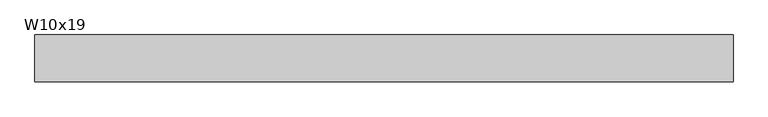
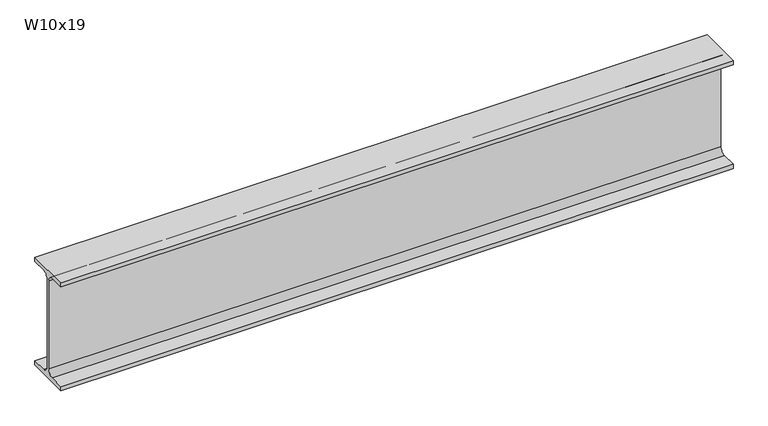
"""IFC4 building model written with IfcOpenShell, lengths in millimetres: beam geometry, RME W-Wide Flange : W10x19."""

from ifc_helpers import new_model, si_unit, point, frame, frame_2d, origin, place, context, project, spatial, polyline, circle_curve, trimmed, segment, composite_curve, outline, extrude, source, transform, mapped, element, save


def w10x19_decb9594(model_context):
    return source(origin(), model_context, "Body", "SweptSolid", [
        extrude(outline(composite_curve([segment(polyline([(51.054, -119.507), (51.054, -129.54), (-51.054, -129.54), (-51.054, -119.507), (-16.9545, -119.507)]), True, "CONTINUOUS"), segment(trimmed(circle_curve(frame_2d((-16.9545, -105.7275)), 13.7795), [point((-16.9545, -119.507))], [point((-3.175, -105.7275))], True, "CARTESIAN"), True, "CONTINUOUS"), segment(polyline([(-3.175, -105.7275), (-3.175, 105.7275)]), True, "CONTINUOUS"), segment(trimmed(circle_curve(frame_2d((-16.9545, 105.7275)), 13.7795), [point((-3.175, 105.7275))], [point((-16.9545, 119.507))], True, "CARTESIAN"), True, "CONTINUOUS"), segment(polyline([(-16.9545, 119.507), (-51.054, 119.507), (-51.054, 129.54), (51.054, 129.54), (51.054, 119.507), (16.9545, 119.507)]), True, "CONTINUOUS"), segment(trimmed(circle_curve(frame_2d((16.9545, 105.7275)), 13.7795), [point((16.9545, 119.507))], [point((3.175, 105.7275))], True, "CARTESIAN"), True, "CONTINUOUS"), segment(polyline([(3.175, 105.7275), (3.175, -105.7275)]), True, "CONTINUOUS"), segment(trimmed(circle_curve(frame_2d((16.9545, -105.7275)), 13.7795), [point((3.175, -105.7275))], [point((16.9545, -119.507))], True, "CARTESIAN"), True, "CONTINUOUS"), segment(polyline([(16.9545, -119.507), (51.054, -119.507)]), True, "CONTINUOUS")], self_intersect=False)), frame((-763.2780813, 0.0, 0.0), z_axis=(1.0, 0.0, 0.0), x_axis=(0.0, 1.0, 0.0)), (0.0, 0.0, 1.0), 1526.5561627),
    ])


if __name__ == "__main__":
    model = new_model("IFC4")
    model_context = context("Model", 3, world=origin())
    ifc_project = project(units=[si_unit("LENGTHUNIT", "METRE", prefix="MILLI")], contexts=[model_context])
    site = spatial("IfcSite", under=ifc_project)
    building = spatial("IfcBuilding", under=site)
    placement = place(None, origin())
    w10x19_shape = w10x19_decb9594(model_context)
    element("IfcBeam", 1, ObjectType="RME W-Wide Flange : W10x19", at=placement, inside=building, context=model_context, shape_type="MappedRepresentation", body=[
        mapped(w10x19_shape, transform((0.0, 0.0, 0.0), x_axis=(1.0, 0.0, 0.0), y_axis=(0.0, 1.0, 0.0), z_axis=(0.0, 0.0, 1.0))),
    ])
    save(model, "model.ifc")

# Revit data of these elements
# Type "RME W-Wide Flange : W10x19"
#   WELD P [instance default] = ""
#   WELD LE [instance default] = ""
#   WELD D [instance default] = ""
#   TOP SECTION SIZE [instance default] = ""
#   TOP SECTION LENGTH [instance default] = ""
#   REMARKS [instance default] = ""
#   REINF TYPE [instance default] = ""
#   Nominal Size = "W24"
#   End Bearing Capacity [instance default] = ""
#   BOT SECTION SIZE [instance default] = ""
#   BOT SECTION LENGTH [instance default] = ""
#   Assembly Code = "B10"
#   W = 19
#   Start Extension Calculation [instance default] = 10' - 0"
#   Start Extension [instance default] = -0' - 0 1/2"
#   End Extension Calculation [instance default] = 10' - 0"
#   End Extension [instance default] = -0' - 0 1/2"
#   Length [instance default] = 5' - 0"
#   bf = 0' - 4.02"
#   d = 0' - 10.2"
#   k = 0' - 0 15/16"
#   k2 = 0' - 0.5425"
#   tf = 0' - 0.395"
#   tw = 0' - 0 1/4"
#   A = 0.0390278 SF
#   Structural Material [instance default] = Metal - Steel - ASTM A992
# Element 1 (IfcBeam, "RME W-Wide Flange : W10x19")
#   Length = 5' - 0.10064"
#   Materials on its faces: "Metal - Steel - ASTM A992"
# Materials
#   "Metal - Steel - ASTM A992": class "Metal", colour RGB 255 128 0, transparency 0
